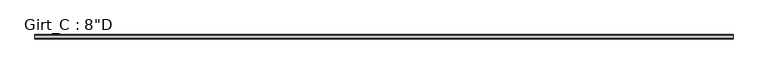
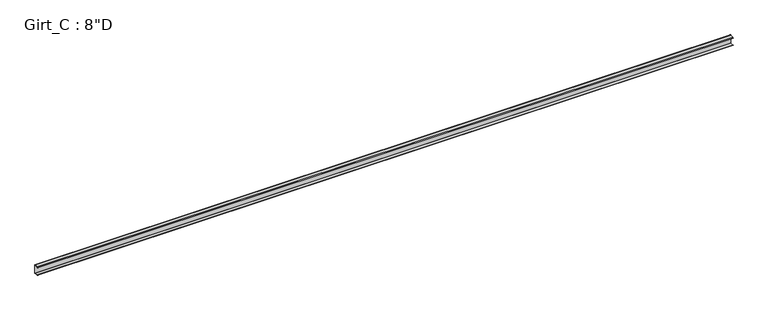
"""IFC4 building model written with IfcOpenShell, lengths in millimetres: beam geometry."""

import ifcopenshell
import ifcopenshell.guid

model = None  # the IFC model being written
_history = None  # IfcOwnerHistory: only IFC2X3 demands one
_inside = {}  # id of a spatial element -> (the spatial element, [elements in it])
_under = {}  # id of a project, library or spatial element -> (it, [spatial elements below it])
_declared = {}  # id of a project -> (the project, [libraries it declares])
_typed = {}  # id of a type object -> (the type object, [elements of that type])
_made_of = {}  # id of a material, layer set ... -> (it, [elements and type objects made of it])


def new_model(schema):
    """Start an empty IFC model of exactly this schema.

    Asked for "IFC4X3", IfcOpenShell would pick the latest addendum, in which some entities
    have other attributes; the version numbers below select the first issue.
    IFC2X3 requires an IfcOwnerHistory on every rooted entity: one is made here for all.
    """
    global model, _history
    if schema == "IFC4X3":
        model = ifcopenshell.file(schema_version=(4, 3, 0, 0))
    else:
        model = ifcopenshell.file(schema=schema)
    _inside.clear()
    _under.clear()
    _declared.clear()
    _typed.clear()
    _made_of.clear()
    _history = None
    if model.schema == "IFC2X3":
        org = make("IfcOrganization", Name="unknown")
        user = make(
            "IfcPersonAndOrganization",
            ThePerson=make("IfcPerson", FamilyName="unknown"),
            TheOrganization=org,
        )
        app = make(
            "IfcApplication",
            ApplicationDeveloper=org,
            Version="unknown",
            ApplicationFullName="unknown",
            ApplicationIdentifier="unknown",
        )
        _history = make(
            "IfcOwnerHistory",
            OwningUser=user,
            OwningApplication=app,
            ChangeAction="ADDED",
            CreationDate=0,
        )
    return model


def make(cls, **values):
    """One entity of the class cls with the attributes given. An attribute that is None is left unset."""
    return model.create_entity(
        cls, **{name: value for name, value in values.items() if value is not None}
    )


def rooted(cls, **values):
    """An entity with a GlobalId (a new one), such as an element, a storey or a relation."""
    return make(cls, GlobalId=ifcopenshell.guid.new(), OwnerHistory=_history, **values)


def si_unit(unit_type, name, prefix=None):
    """IfcSIUnit, for example si_unit("LENGTHUNIT", "METRE", prefix="MILLI")."""
    return make("IfcSIUnit", UnitType=unit_type, Prefix=prefix, Name=name)


def assignment(units):
    """IfcUnitAssignment: the units of a project."""
    return None if units is None else make("IfcUnitAssignment", Units=units)


def point(xyz):
    """IfcCartesianPoint."""
    return None if xyz is None else make("IfcCartesianPoint", Coordinates=xyz)


def direction(xyz):
    """IfcDirection."""
    return None if xyz is None else make("IfcDirection", DirectionRatios=xyz)


def frame(location, z_axis=None, x_axis=None):
    """IfcAxis2Placement3D, a coordinate frame: its origin and axes. An axis left out is left unset."""
    return make(
        "IfcAxis2Placement3D",
        Location=point(location),
        Axis=direction(z_axis),
        RefDirection=direction(x_axis),
    )


def frame_2d(location, x_axis=None):
    """IfcAxis2Placement2D, a coordinate frame in the plane: its origin and x axis."""
    return make(
        "IfcAxis2Placement2D", Location=point(location), RefDirection=direction(x_axis)
    )


def origin():
    """The frame at (0, 0, 0) with its axes left unset."""
    return frame((0.0, 0.0, 0.0))


def place(relative_to, where):
    """IfcLocalPlacement: puts the frame where relative to a parent placement (None: the world)."""
    return make(
        "IfcLocalPlacement", PlacementRelTo=relative_to, RelativePlacement=where
    )


def context(
    kind, dimensions, precision=None, world=None, true_north=None, identifier=None
):
    """IfcGeometricRepresentationContext, for example the 3D "Model" context."""
    return make(
        "IfcGeometricRepresentationContext",
        ContextIdentifier=identifier,
        ContextType=kind,
        CoordinateSpaceDimension=dimensions,
        Precision=precision,
        WorldCoordinateSystem=world,
        TrueNorth=true_north,
    )


def project(units=None, contexts=None):
    """IfcProject with its units and contexts."""
    return rooted(
        "IfcProject",
        Name="project",
        RepresentationContexts=contexts,
        UnitsInContext=assignment(units),
    )


def spatial(cls, under=None, at=None, **own):
    """A site, building, storey or space (cls), placed at a placement, below another one or the project."""
    s = rooted(cls, ObjectPlacement=at, **own)
    if under is not None:
        _under.setdefault(under.id(), (under, []))[1].append(s)
    return s


def polyline(points):
    """IfcPolyline through the points."""
    return make("IfcPolyline", Points=[point(p) for p in points])


def circle_curve(where, radius):
    """IfcCircle in the frame where."""
    return make("IfcCircle", Position=where, Radius=radius)


def trimmed(basis, trim1, trim2, sense, master):
    """IfcTrimmedCurve: the piece of a basis curve between two trims."""
    return make(
        "IfcTrimmedCurve",
        BasisCurve=basis,
        Trim1=trim1,
        Trim2=trim2,
        SenseAgreement=sense,
        MasterRepresentation=master,
    )


def segment(curve, same_sense, transition):
    """IfcCompositeCurveSegment."""
    return make(
        "IfcCompositeCurveSegment",
        Transition=transition,
        SameSense=same_sense,
        ParentCurve=curve,
    )


def composite_curve(segments, self_intersect=None):
    """IfcCompositeCurve: segments joined end to end."""
    return make("IfcCompositeCurve", Segments=segments, SelfIntersect=self_intersect)


def outline(outer, holes=None, kind="AREA"):
    """IfcArbitraryClosedProfileDef: a profile drawn as a closed curve; with holes, ...WithVoids."""
    if holes is None:
        return make("IfcArbitraryClosedProfileDef", ProfileType=kind, OuterCurve=outer)
    return make(
        "IfcArbitraryProfileDefWithVoids",
        ProfileType=kind,
        OuterCurve=outer,
        InnerCurves=holes,
    )


def extrude(swept, where, along, depth):
    """IfcExtrudedAreaSolid: the profile swept, set in the frame where, extruded along a direction by depth."""
    return make(
        "IfcExtrudedAreaSolid",
        SweptArea=swept,
        Position=where,
        ExtrudedDirection=direction(along),
        Depth=depth,
    )


def shape(context_of_items, identifier, shape_type, items):
    """IfcShapeRepresentation: the items that make up one representation, for example the "Body"."""
    return make(
        "IfcShapeRepresentation",
        ContextOfItems=context_of_items,
        RepresentationIdentifier=identifier,
        RepresentationType=shape_type,
        Items=items,
    )


def source(mapping_origin, context_of_items, identifier, shape_type, items):
    """IfcRepresentationMap: a shape defined once, which mapped items show again and again."""
    return make(
        "IfcRepresentationMap",
        MappingOrigin=mapping_origin,
        MappedRepresentation=shape(context_of_items, identifier, shape_type, items),
    )


def transform(
    local_origin,
    x_axis=None,
    y_axis=None,
    z_axis=None,
    scale=None,
    scale2=None,
    scale3=None,
    uniform=True,
):
    """IfcCartesianTransformationOperator3D, or its non-uniform kind. x_axis, y_axis, z_axis: its Axis1, 2, 3."""
    if uniform:
        return make(
            "IfcCartesianTransformationOperator3D",
            Axis1=direction(x_axis),
            Axis2=direction(y_axis),
            LocalOrigin=point(local_origin),
            Scale=scale,
            Axis3=direction(z_axis),
        )
    return make(
        "IfcCartesianTransformationOperator3DnonUniform",
        Axis1=direction(x_axis),
        Axis2=direction(y_axis),
        LocalOrigin=point(local_origin),
        Scale=scale,
        Axis3=direction(z_axis),
        Scale2=scale2,
        Scale3=scale3,
    )


def mapped(mapping_source, mapping_target):
    """IfcMappedItem: shows the shape of a source again, moved by a transform."""
    return make(
        "IfcMappedItem", MappingSource=mapping_source, MappingTarget=mapping_target
    )


def made_of(thing, what):
    """Note that an element or type object is made of a material, layer set ...; save() writes the relation."""
    if what is not None:
        _made_of.setdefault(what.id(), (what, []))[1].append(thing)
    return thing


def element(
    cls,
    number,
    at=None,
    inside=None,
    cuts=None,
    type_object=None,
    material=None,
    context=None,
    identifier="Body",
    shape_type=None,
    held_by="IfcProductDefinitionShape",
    body=None,
    shapes=None,
    **own,
):
    """One element of the class cls, such as IfcWall. Its Tag is "e" and its number.

    at: its placement. inside: the storey or other place that contains it. cuts: it is an
    opening in that element (IfcRelVoidsElement). A single representation is given by context,
    identifier, shape_type and body (its items); several are given by shapes. held_by: the class
    of the entity that holds the representations. save() writes the other relations.
    """
    e = rooted(cls, Tag="e%d" % number, ObjectPlacement=at, **own)
    if body is not None:
        shapes = [shape(context, identifier, shape_type, body)]
    if shapes is not None:
        e.Representation = make(held_by, Representations=shapes)
    if inside is not None:
        _inside.setdefault(inside.id(), (inside, []))[1].append(e)
    if cuts is not None:
        rooted(
            "IfcRelVoidsElement", RelatingBuildingElement=cuts, RelatedOpeningElement=e
        )
    if type_object is not None:
        _typed.setdefault(type_object.id(), (type_object, []))[1].append(e)
    return made_of(e, material)


def aggregate(whole, parts):
    """IfcRelAggregates: a whole, such as a stair, and the parts it consists of."""
    return rooted("IfcRelAggregates", RelatingObject=whole, RelatedObjects=parts)


def save(model, path):
    """Write the relations noted so far, then the file.

    IfcRelAggregates (storeys below a building ...), IfcRelContainedInSpatialStructure (elements
    in a storey), IfcRelDefinesByType, IfcRelAssociatesMaterial and IfcRelDeclares: one each for
    every whole, place, type object, material and project.
    """
    for whole, parts in _under.values():
        aggregate(whole, parts)
    for where, things in _inside.values():
        rooted(
            "IfcRelContainedInSpatialStructure",
            RelatedElements=things,
            RelatingStructure=where,
        )
    for kind, things in _typed.values():
        rooted("IfcRelDefinesByType", RelatedObjects=things, RelatingType=kind)
    for what, things in _made_of.values():
        rooted("IfcRelAssociatesMaterial", RelatedObjects=things, RelatingMaterial=what)
    for by, libraries in _declared.values():
        rooted("IfcRelDeclares", RelatingContext=by, RelatedDefinitions=libraries)
    model.write(path)


def beam_22635dde(model_context):
    return source(origin(), model_context, "Body", "SweptSolid", [
        extrude(outline(composite_curve([segment(polyline([(-87.5109375, 101.6), (-3.3734375, 101.6)]), True, "CONTINUOUS"), segment(trimmed(circle_curve(frame_2d((-3.3734375, 96.8375)), 4.7625), [point((-3.3734375, 101.6))], [point((1.3890625, 96.8375))], False, "CARTESIAN"), True, "CONTINUOUS"), segment(polyline([(1.3890625, 96.8375), (1.3890625, -96.8375)]), True, "CONTINUOUS"), segment(trimmed(circle_curve(frame_2d((-3.3734375, -96.8375)), 4.7625), [point((1.3890625, -96.8375))], [point((-3.3734375, -101.6))], False, "CARTESIAN"), True, "CONTINUOUS"), segment(polyline([(-3.3734375, -101.6), (-87.5109375, -101.6), (-99.7792647, -86.979177), (-97.6510975, -85.1934327), (-86.2154765, -98.821875), (-3.2694106, -98.821875)]), True, "CONTINUOUS"), segment(trimmed(circle_curve(frame_2d((-3.3748024, -96.8389339)), 1.9857399), [point((-3.2694106, -98.821875))], [point((-1.3890625, -96.8389339))], True, "CARTESIAN"), True, "CONTINUOUS"), segment(polyline([(-1.3890625, -96.8389339), (-1.3890625, 96.8381931)]), True, "CONTINUOUS"), segment(trimmed(circle_curve(frame_2d((-3.3741066, 96.8381931)), 1.9850441), [point((-1.3890625, 96.8381931))], [point((-3.3005807, 98.821875))], True, "CARTESIAN"), True, "CONTINUOUS"), segment(polyline([(-3.3005807, 98.821875), (-86.2154765, 98.821875), (-97.6278742, 85.221109), (-99.7560415, 87.0068534), (-87.5109375, 101.6)]), True, "CONTINUOUS")], self_intersect=False)), frame((-7996.2976659, 0.0, 0.0), z_axis=(1.0, 0.0, 0.0), x_axis=(0.0, 1.0, 0.0)), (0.0, 0.0, 1.0), 15992.5953317),
    ])


if __name__ == "__main__":
    model = new_model("IFC4")
    model_context = context("Model", 3, world=origin())
    ifc_project = project(units=[si_unit("LENGTHUNIT", "METRE", prefix="MILLI")], contexts=[model_context])
    site = spatial("IfcSite", under=ifc_project)
    building = spatial("IfcBuilding", under=site)
    placement = place(None, origin())
    beam_shape = beam_22635dde(model_context)
    element("IfcBeam", 1, ObjectType="Girt_C : 8\"D", at=placement, inside=building, context=model_context, shape_type="MappedRepresentation", body=[
        mapped(beam_shape, transform((0.0, 0.0, 0.0), x_axis=(1.0, 0.0, 0.0), y_axis=(0.0, 1.0, 0.0), z_axis=(0.0, 0.0, 1.0))),
    ])
    save(model, "model.ifc")

# Revit data of these elements
# Type "Girt_C : 8\"D"
#   half leg = 0' - 1 3/4"
#   Web_Thickness = 0' - 0 7/64"
#   Length [instance default] = 10' - 0"
#   Leg_1 = 0' - 3 1/2"
#   Height = 0' - 8"
#   Structural Material [instance default] = none
# Element 1 (IfcBeam, "Girt_C : 8\"D")
#   Structural Material = GALVANIZED 'CEE' SECTION (8.0x3.5C - SEE STRUCT. DWGS)
#   Materials on its faces: "GALVANIZED 'CEE' SECTION (8.0x3.5C - SEE STRUCT. DWGS)"
# Materials
#   "GALVANIZED 'CEE' SECTION (8.0x3.5C - SEE STRUCT. DWGS)": class "Metal", colour RGB 137 146 153, transparency 0, Description = "Steel, mill finish", Cost = 0
